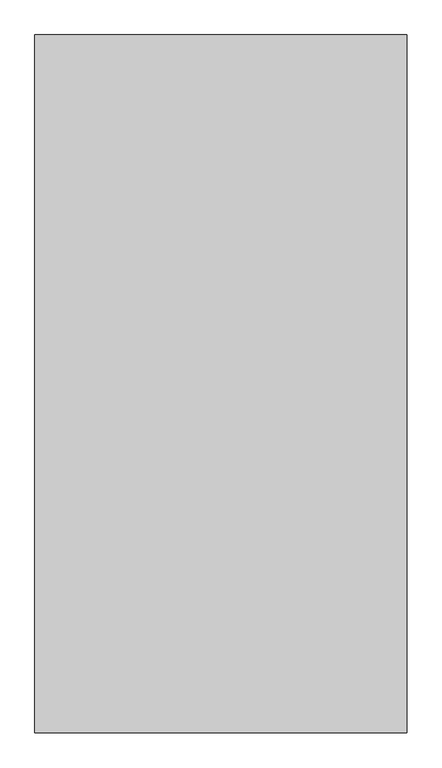
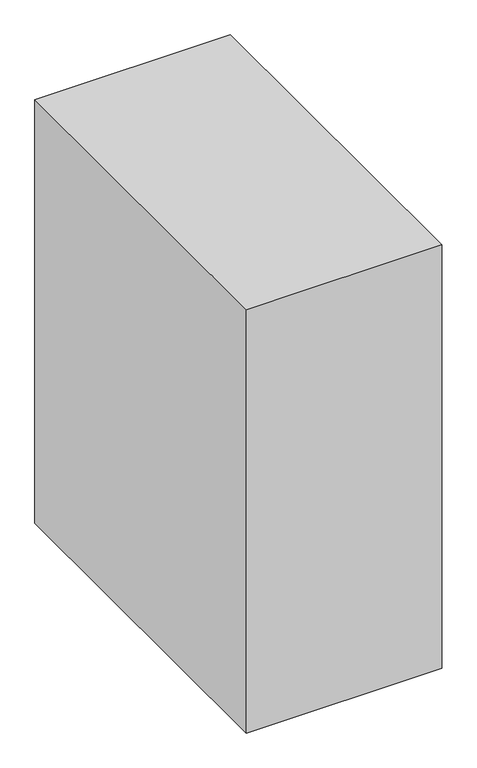
"""IFC4 building model written with IfcOpenShell, lengths in millimetres: proxy geometry, Space Planning Box_hec : Space Planning Box_hec."""

from ifc_helpers import new_model, si_unit, origin, origin_with_axes, place, context, project, spatial, polyline, outline, extrude, source, transform, mapped, element, save


def generic_models_570012e4(model_context):
    return source(origin(), model_context, "Body", "SweptSolid", [
        extrude(outline(polyline([(1200.0, 2250.0), (1200.0, -2250.0), (-1200.0, -2250.0), (-1200.0, 2250.0), (1200.0, 2250.0)])), origin_with_axes(), (0.0, 0.0, 1.0), 5500.0),
    ])


if __name__ == "__main__":
    model = new_model("IFC4")
    model_context = context("Model", 3, world=origin())
    ifc_project = project(units=[si_unit("LENGTHUNIT", "METRE", prefix="MILLI")], contexts=[model_context])
    site = spatial("IfcSite", under=ifc_project)
    building = spatial("IfcBuilding", under=site)
    placement = place(None, origin())
    generic_models_shape = generic_models_570012e4(model_context)
    element("IfcBuildingElementProxy", 1, Name="Space Planning Box_hec : Space Planning Box_hec", ObjectType="Space Planning Box_hec : Space Planning Box_hec", at=placement, inside=building, context=model_context, shape_type="MappedRepresentation", body=[
        mapped(generic_models_shape, transform((0.0, 0.0, 0.0), x_axis=(1.0, 0.0, 0.0), y_axis=(0.0, 1.0, 0.0), z_axis=(0.0, 0.0, 1.0))),
    ])
    save(model, "model.ifc")

# Revit data of these elements
# Type "Space Planning Box_hec : Space Planning Box_hec"
#   Type Comments = "..."
#   Room Name [instance default] = "?"
#   Interior Finish [instance default] = ""
#   Exterior Finish [instance default] = ""
#   Department [instance default] = ""
#   Assembly Code = "..."
#   ceiling height [instance default] = 0
#   Width [instance default] = 1524 mm
#   Program Area [instance default] = 0.00 m²
#   Length [instance default] = 1524 mm
#   Height [instance default] = 1524 mm
#   Area [instance default] = 2.32258 m²
#   Fill Color [instance default] = Cyan
#   Default Elevation = 0
# Element 1 (IfcBuildingElementProxy, "Space Planning Box_hec : Space Planning Box_hec")
#   Room Name = "Duct Shaft"
#   Exterior Finish = "N/A..N/A,,EW2..N/A..N/A"
#   Department = "PATHV3"
#   Width = 2400 mm
#   Program Area = 10.80 m²
#   Length = 4500 mm
#   Height = 5500 mm
#   Area = 10.80 m²
#   Fill Color = Lavender
#   Materials on its faces: "Lavender"
# Materials
#   "Cyan": class "Generic", colour RGB 0 255 255, transparency 0.2, Cost = 0
#   "Lavender": class "Generic", colour RGB 186 85 211, transparency 0.2, Cost = 0
